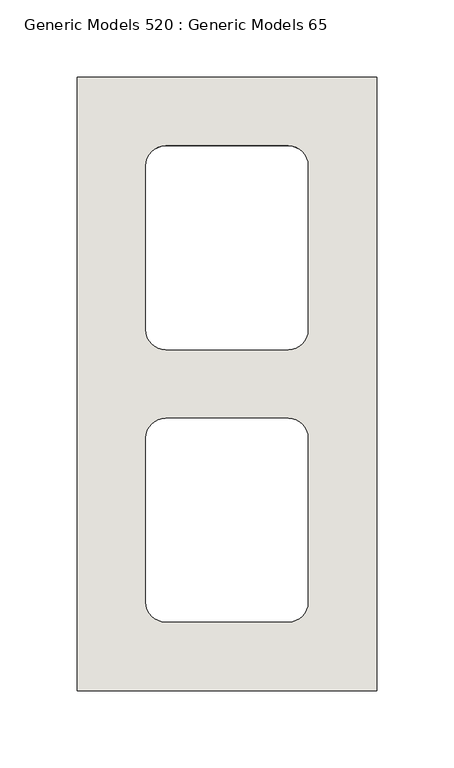
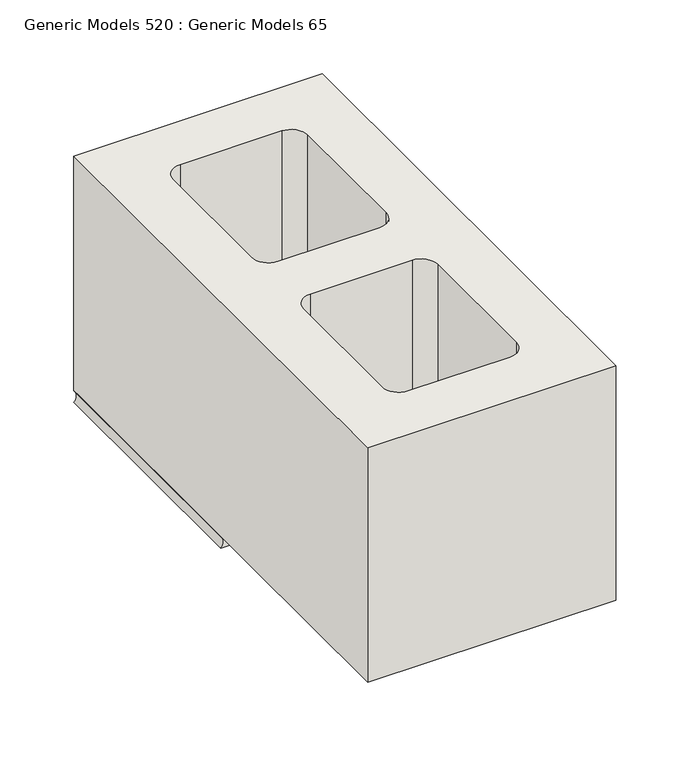
"""IFC4 building model written with IfcOpenShell, lengths in millimetres: wall geometry, Generic Models 520 : Generic Models 65."""

from ifc_helpers import new_model, si_unit, point, frame, frame_2d, origin, place, context, project, spatial, polyline, circle_curve, trimmed, segment, composite_curve, outline, extrude, source, transform, mapped, element, save
from ifc_brep_helpers import plane_surface, revolved_surface, advanced_brep


def generic_models_520_generic_models_65_cdbb6447(model_context):
    return source(origin(), model_context, "Body", "SolidModel", [
        advanced_brep(
        [(428979.0125, 503.2375, 1838.325), (428785.3375, 503.2375, 1838.325), (428785.3375, 503.2375, 1828.8), (428979.0125, 503.2375, 1828.8), (428979.0125, 701.675, 1838.325), (428979.0125, 701.675, 1828.8), (428785.3375, 701.675, 1828.8), (428785.3375, 701.675, 1838.325), (428934.5625, 538.1625, 1838.325), (428921.8625, 525.4625, 1838.325), (428842.4875, 525.4625, 1838.325), (428829.7875, 538.1625, 1838.325), (428829.7875, 644.525, 1838.325), (428842.4875, 657.225, 1838.325), (428921.8625, 657.225, 1838.325), (428934.5625, 644.525, 1838.325), (428921.8625, 525.4625, 1828.8), (428934.5625, 538.1625, 1828.8), (428842.4875, 525.4625, 1828.8), (428829.7875, 538.1625, 1828.8), (428829.7875, 644.525, 1828.8), (428842.4875, 657.225, 1828.8), (428921.8625, 657.225, 1828.8), (428934.5625, 644.525, 1828.8)],
        [
            (0, 1),
            (1, 2, circle_curve(frame((428780.4545028, 503.2375, 1833.5625), z_axis=(0.0, 1.0, 0.0), x_axis=(1.0, 0.0, 0.0)), 6.8209287)),
            (2, 3),
            (3, 0, circle_curve(frame((428983.8954972, 503.2375, 1833.5625), z_axis=(0.0, 1.0, 0.0), x_axis=(-1.0, 0.0, 0.0)), 6.8209287)),
            (4, 5, circle_curve(frame((428983.8954972, 701.675, 1833.5625), z_axis=(0.0, -1.0, 0.0), x_axis=(-1.0, 0.0, 0.0)), 6.8209287)),
            (5, 6),
            (6, 7, circle_curve(frame((428780.4545028, 701.675, 1833.5625), z_axis=(0.0, -1.0, 0.0), x_axis=(1.0, 0.0, 0.0)), 6.8209287)),
            (7, 4),
            (0, 4),
            (7, 1),
            (8, 9, circle_curve(frame((428921.8625, 538.1625, 1838.325), z_axis=(0.0, 0.0, -1.0), x_axis=(-1.0, 0.0, 0.0)), 12.7)),
            (9, 10),
            (10, 11, circle_curve(frame((428842.4875, 538.1625, 1838.325), z_axis=(0.0, 0.0, -1.0), x_axis=(-1.0, 0.0, 0.0)), 12.7)),
            (11, 12),
            (12, 13, circle_curve(frame((428842.4875, 644.525, 1838.325), z_axis=(0.0, 0.0, -1.0), x_axis=(-1.0, 0.0, 0.0)), 12.7)),
            (13, 14),
            (14, 15, circle_curve(frame((428921.8625, 644.525, 1838.325), z_axis=(0.0, 0.0, -1.0), x_axis=(-1.0, 0.0, 0.0)), 12.7)),
            (15, 8),
            (16, 9),
            (8, 17),
            (17, 16, circle_curve(frame((428921.8625, 538.1625, 1828.8), z_axis=(0.0, 0.0, -1.0), x_axis=(-1.0, 0.0, 0.0)), 12.7)),
            (16, 18),
            (18, 10),
            (18, 19, circle_curve(frame((428842.4875, 538.1625, 1828.8), z_axis=(0.0, 0.0, -1.0), x_axis=(-1.0, 0.0, 0.0)), 12.7)),
            (19, 11),
            (19, 20),
            (20, 12),
            (20, 21, circle_curve(frame((428842.4875, 644.525, 1828.8), z_axis=(0.0, 0.0, -1.0), x_axis=(-1.0, 0.0, 0.0)), 12.7)),
            (21, 13),
            (21, 22),
            (22, 14),
            (22, 23, circle_curve(frame((428921.8625, 644.525, 1828.8), z_axis=(0.0, 0.0, -1.0), x_axis=(-1.0, 0.0, 0.0)), 12.7)),
            (23, 15),
            (23, 17),
            (6, 2),
            (5, 3),
        ],
        [
            plane_surface(frame((428882.175, 503.2375, 1838.721875), z_axis=(0.0, -1.0, 0.0), x_axis=(0.0, 0.0, 1.0))),
            plane_surface(frame((428882.175, 701.675, 1838.721875), z_axis=(0.0, 1.0, 0.0), x_axis=(0.0, 0.0, 1.0))),
            plane_surface(frame((428979.0125, 503.2375, 1838.325), z_axis=(0.0, 0.0, 1.0), x_axis=(0.0, 1.0, 0.0))),
            revolved_surface(polyline([(428909.1625, 538.1625, 1838.325), (428909.1625, 538.1625, 1828.8)]), (428921.8625, 538.1625, 2022.475), (0.0, 0.0, 1.0)),
            plane_surface(frame((428842.4875, 525.4625, 2022.475), z_axis=(0.0, 1.0, 0.0), x_axis=(0.0, 0.0, -1.0))),
            revolved_surface(polyline([(428829.7875, 538.1625, 1838.325), (428829.7875, 538.1625, 1828.8)]), (428842.4875, 538.1625, 2022.475), (0.0, 0.0, 1.0)),
            plane_surface(frame((428829.7875, 644.525, 2022.475), z_axis=(1.0, 0.0, 0.0), x_axis=(0.0, 0.0, -1.0))),
            revolved_surface(polyline([(428829.7875, 644.525, 1838.325), (428829.7875, 644.525, 1828.8)]), (428842.4875, 644.525, 2022.475), (0.0, 0.0, 1.0)),
            plane_surface(frame((428921.8625, 657.225, 2022.475), z_axis=(0.0, -1.0, 0.0), x_axis=(0.0, 0.0, -1.0))),
            revolved_surface(polyline([(428909.1625, 644.525, 1838.325), (428909.1625, 644.525, 1828.8)]), (428921.8625, 644.525, 2022.475), (0.0, 0.0, 1.0)),
            plane_surface(frame((428934.5625, 538.1625, 2022.475), z_axis=(-1.0, 0.0, 0.0), x_axis=(0.0, 0.0, -1.0))),
            revolved_surface(polyline([(428787.2754315, 701.675, 1833.5625), (428787.2754315, 503.2375, 1833.5625)]), (428780.4545028, 503.2375, 1833.5625), (0.0, 1.0, 0.0)),
            plane_surface(frame((428785.3375, 503.2375, 1828.8), z_axis=(0.0, 0.0, -1.0), x_axis=(0.0, 1.0, 0.0))),
            revolved_surface(polyline([(428977.07456850004, 701.675, 1833.5625), (428977.07456850004, 503.2375, 1833.5625)]), (428983.8954972, 503.2375, 1833.5625), (0.0, 1.0, 0.0)),
        ],
        [
            (0, [[1, 2, 3, 4]]),
            (1, [[5, 6, 7, 8]]),
            (2, [[-1, 9, -8, 10], [11, 12, 13, 14, 15, 16, 17, 18]]),
            (3, [[19, -11, 20, 21]]),
            (4, [[-19, 22, 23, -12]]),
            (5, [[-23, 24, 25, -13]]),
            (6, [[-25, 26, 27, -14]]),
            (7, [[-27, 28, 29, -15]]),
            (8, [[-29, 30, 31, -16]]),
            (9, [[-31, 32, 33, -17]]),
            (10, [[-33, 34, -20, -18]]),
            (11, [[-2, -10, -7, 35]]),
            (12, [[-3, -35, -6, 36], [-21, -34, -32, -30, -28, -26, -24, -22]]),
            (13, [[-4, -36, -5, -9]]),
        ],
    ),
        extrude(outline(polyline([(428979.0125, 304.8), (428785.3375, 304.8), (428785.3375, 701.675), (428979.0125, 701.675), (428979.0125, 304.8)]), holes=[composite_curve([segment(polyline([(428934.5625, 538.1625), (428934.5625, 644.525)]), True, "CONTINUOUS"), segment(trimmed(circle_curve(frame_2d((428921.8625, 644.525)), 12.7), [point((428934.5625, 644.525))], [point((428921.8625, 657.225))], True, "CARTESIAN"), True, "CONTINUOUS"), segment(polyline([(428921.8625, 657.225), (428842.4875, 657.225)]), True, "CONTINUOUS"), segment(trimmed(circle_curve(frame_2d((428842.4875, 644.525)), 12.7), [point((428842.4875, 657.225))], [point((428829.7875, 644.525))], True, "CARTESIAN"), True, "CONTINUOUS"), segment(polyline([(428829.7875, 644.525), (428829.7875, 538.1625)]), True, "CONTINUOUS"), segment(trimmed(circle_curve(frame_2d((428842.4875, 538.1625)), 12.7), [point((428829.7875, 538.1625))], [point((428842.4875, 525.4625))], True, "CARTESIAN"), True, "CONTINUOUS"), segment(polyline([(428842.4875, 525.4625), (428921.8625, 525.4625)]), True, "CONTINUOUS"), segment(trimmed(circle_curve(frame_2d((428921.8625, 538.1625)), 12.7), [point((428921.8625, 525.4625))], [point((428934.5625, 538.1625))], True, "CARTESIAN"), True, "CONTINUOUS")], self_intersect=False), composite_curve([segment(polyline([(428829.7875, 468.3125), (428829.7875, 361.95)]), True, "CONTINUOUS"), segment(trimmed(circle_curve(frame_2d((428842.4875, 361.95)), 12.7), [point((428829.7875, 361.95))], [point((428842.4875, 349.25))], True, "CARTESIAN"), True, "CONTINUOUS"), segment(polyline([(428842.4875, 349.25), (428921.8625, 349.25)]), True, "CONTINUOUS"), segment(trimmed(circle_curve(frame_2d((428921.8625, 361.95)), 12.7), [point((428921.8625, 349.25))], [point((428934.5625, 361.95))], True, "CARTESIAN"), True, "CONTINUOUS"), segment(polyline([(428934.5625, 361.95), (428934.5625, 468.3125)]), True, "CONTINUOUS"), segment(trimmed(circle_curve(frame_2d((428921.8625, 468.3125)), 12.7), [point((428934.5625, 468.3125))], [point((428921.8625, 481.0125))], True, "CARTESIAN"), True, "CONTINUOUS"), segment(polyline([(428921.8625, 481.0125), (428842.4875, 481.0125)]), True, "CONTINUOUS"), segment(trimmed(circle_curve(frame_2d((428842.4875, 468.3125)), 12.7), [point((428842.4875, 481.0125))], [point((428829.7875, 468.3125))], True, "CARTESIAN"), True, "CONTINUOUS")], self_intersect=False)]), frame((0.0, 0.0, 1838.325), z_axis=(0.0, 0.0, 1.0), x_axis=(1.0, 0.0, 0.0)), (0.0, 0.0, 1.0), 193.675),
    ])


if __name__ == "__main__":
    model = new_model("IFC4")
    model_context = context("Model", 3, world=origin())
    ifc_project = project(units=[si_unit("LENGTHUNIT", "METRE", prefix="MILLI")], contexts=[model_context])
    site = spatial("IfcSite", under=ifc_project)
    building = spatial("IfcBuilding", under=site)
    placement = place(None, origin())
    generic_models_520_generic_models_65_shape = generic_models_520_generic_models_65_cdbb6447(model_context)
    element("IfcWall", 1, ObjectType="Generic Models 520 : Generic Models 65", at=placement, inside=building, context=model_context, shape_type="MappedRepresentation", body=[
        mapped(generic_models_520_generic_models_65_shape, transform((0.0, 0.0, 0.0), x_axis=(1.0, 0.0, 0.0), y_axis=(0.0, 1.0, 0.0), z_axis=(0.0, 0.0, 1.0))),
    ])
    save(model, "model.ifc")

# Revit data of these elements
# Element 1 (IfcWall, "Generic Models 520 : Generic Models 65")
#   Materials on its faces: "CMU (SEE 'WALL TAG' FOR SIZE)", "MORTAR JOINT"
# Materials
#   "CMU (SEE 'WALL TAG' FOR SIZE)": class "Masonry", colour RGB 203 203 199, transparency 0, Description = "Concrete masonry units", Cost = 0
#   "MORTAR JOINT": class "Generic", colour RGB 120 120 120, transparency 0, Cost = 0
